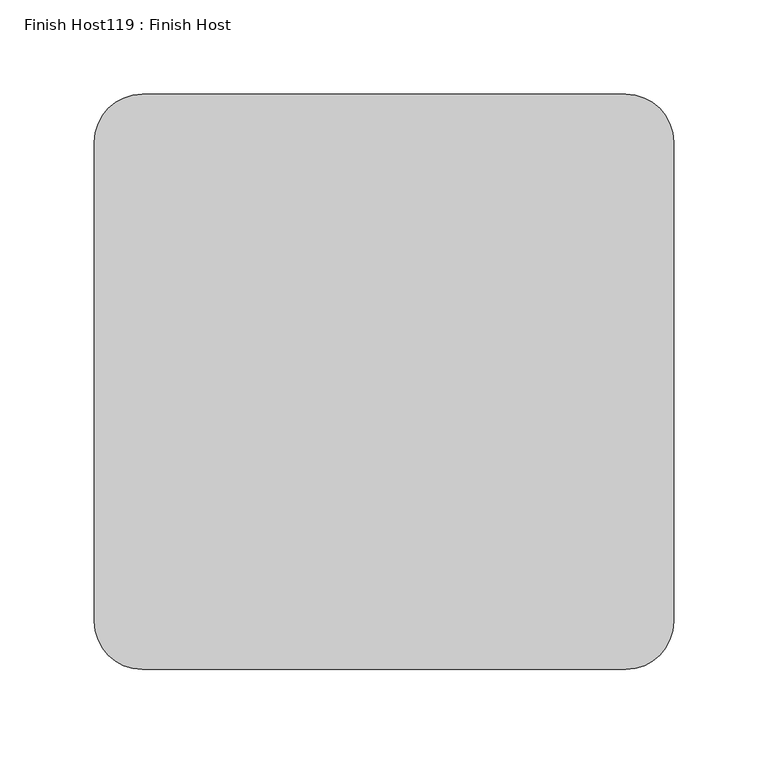
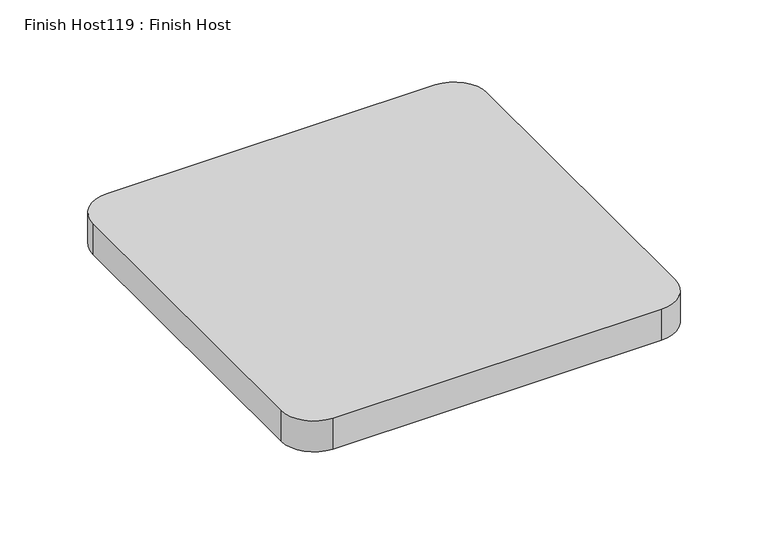
"""IFC4 building model written with IfcOpenShell, lengths in millimetres: proxy geometry, Finish Host119 : Finish Host."""

from ifc_helpers import new_model, si_unit, point, frame_2d, origin, origin_with_axes, place, context, project, spatial, polyline, circle_curve, trimmed, segment, composite_curve, outline, extrude, source, transform, mapped, element, save


def finish_host119_finish_host_e573546b(model_context):
    return source(origin(), model_context, "Body", "SweptSolid", [
        extrude(outline(composite_curve([segment(polyline([(-799.2083644, 3462.3960864), (-799.2083644, 3716.3960864)]), True, "CONTINUOUS"), segment(trimmed(circle_curve(frame_2d((-773.8083644, 3716.3960864)), 25.4), [point((-799.2083644, 3716.3960864))], [point((-773.8083644, 3741.7960864))], False, "CARTESIAN"), True, "CONTINUOUS"), segment(polyline([(-773.8083644, 3741.7960864), (-517.7842816, 3741.7960864)]), True, "CONTINUOUS"), segment(trimmed(circle_curve(frame_2d((-517.7842816, 3716.3960864)), 25.4), [point((-517.7842816, 3741.7960864))], [point((-492.3842816, 3716.3960864))], False, "CARTESIAN"), True, "CONTINUOUS"), segment(polyline([(-492.3842816, 3716.3960864), (-492.3842816, 3462.3960864)]), True, "CONTINUOUS"), segment(trimmed(circle_curve(frame_2d((-517.7842816, 3462.3960864)), 25.4), [point((-492.3842816, 3462.3960864))], [point((-517.7842816, 3436.9960864))], False, "CARTESIAN"), True, "CONTINUOUS"), segment(polyline([(-517.7842816, 3436.9960864), (-773.8083644, 3436.9960864)]), True, "CONTINUOUS"), segment(trimmed(circle_curve(frame_2d((-773.8083644, 3462.3960864)), 25.4), [point((-773.8083644, 3436.9960864))], [point((-799.2083644, 3462.3960864))], False, "CARTESIAN"), True, "CONTINUOUS")], self_intersect=False)), origin_with_axes(), (0.0, 0.0, 1.0), 25.4),
    ])


if __name__ == "__main__":
    model = new_model("IFC4")
    model_context = context("Model", 3, world=origin())
    ifc_project = project(units=[si_unit("LENGTHUNIT", "METRE", prefix="MILLI")], contexts=[model_context])
    site = spatial("IfcSite", under=ifc_project)
    building = spatial("IfcBuilding", under=site)
    placement = place(None, origin())
    finish_host119_finish_host_shape = finish_host119_finish_host_e573546b(model_context)
    element("IfcBuildingElementProxy", 1, Name="Finish Host119 : Finish Host", ObjectType="Finish Host119 : Finish Host", at=placement, inside=building, context=model_context, shape_type="MappedRepresentation", body=[
        mapped(finish_host119_finish_host_shape, transform((0.0, 0.0, 0.0), x_axis=(1.0, 0.0, 0.0), y_axis=(0.0, 1.0, 0.0), z_axis=(0.0, 0.0, 1.0))),
    ])
    save(model, "model.ifc")

# Revit data of these elements
# Type "Finish Host119 : Finish Host"
#   Panel Material = Fabric - Teknion - R384 - Rationale - Abstract
# Element 1 (IfcBuildingElementProxy, "Finish Host119 : Finish Host")
#   Materials on its faces: "Fabric - Teknion - R384 - Rationale - Abstract"
# Materials
#   "Fabric - Teknion - R384 - Rationale - Abstract": class "Fabric", colour RGB 50 50 48, transparency 0, Model = "R384", Manufacturer = "Teknion Studios", URL = "http://www.teknionstudio.com/", Description = "Abstract Rationale", Cost = 0
